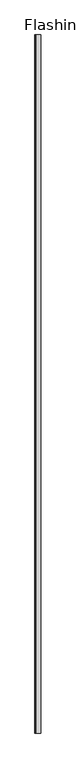
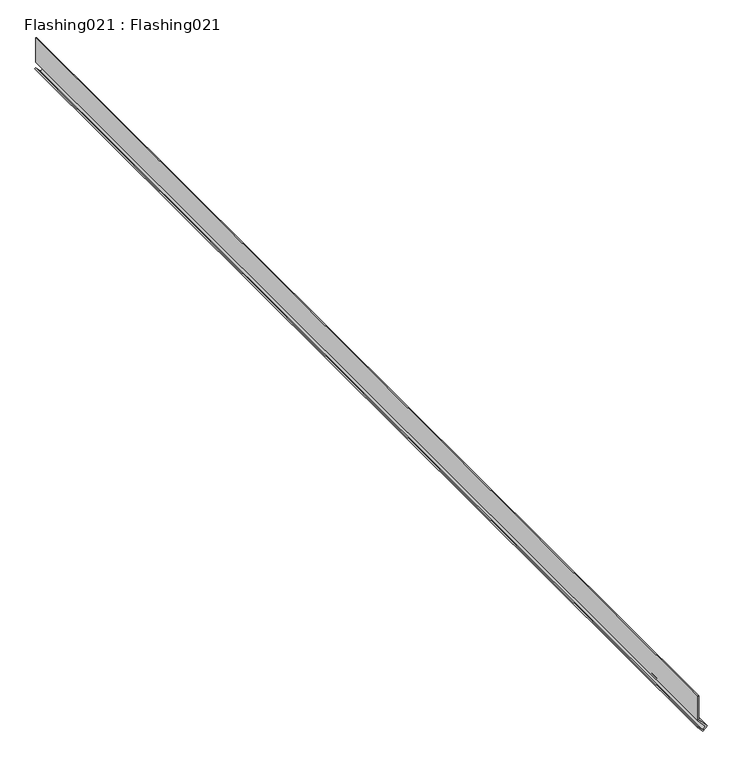
"""IFC4 building model written with IfcOpenShell, lengths in millimetres: proxy geometry, Flashing021 : Flashing021."""

import ifcopenshell
import ifcopenshell.guid

model = None  # the IFC model being written
_history = None  # IfcOwnerHistory: only IFC2X3 demands one
_inside = {}  # id of a spatial element -> (the spatial element, [elements in it])
_under = {}  # id of a project, library or spatial element -> (it, [spatial elements below it])
_declared = {}  # id of a project -> (the project, [libraries it declares])
_typed = {}  # id of a type object -> (the type object, [elements of that type])
_made_of = {}  # id of a material, layer set ... -> (it, [elements and type objects made of it])


def new_model(schema):
    """Start an empty IFC model of exactly this schema.

    Asked for "IFC4X3", IfcOpenShell would pick the latest addendum, in which some entities
    have other attributes; the version numbers below select the first issue.
    IFC2X3 requires an IfcOwnerHistory on every rooted entity: one is made here for all.
    """
    global model, _history
    if schema == "IFC4X3":
        model = ifcopenshell.file(schema_version=(4, 3, 0, 0))
    else:
        model = ifcopenshell.file(schema=schema)
    _inside.clear()
    _under.clear()
    _declared.clear()
    _typed.clear()
    _made_of.clear()
    _history = None
    if model.schema == "IFC2X3":
        org = make("IfcOrganization", Name="unknown")
        user = make(
            "IfcPersonAndOrganization",
            ThePerson=make("IfcPerson", FamilyName="unknown"),
            TheOrganization=org,
        )
        app = make(
            "IfcApplication",
            ApplicationDeveloper=org,
            Version="unknown",
            ApplicationFullName="unknown",
            ApplicationIdentifier="unknown",
        )
        _history = make(
            "IfcOwnerHistory",
            OwningUser=user,
            OwningApplication=app,
            ChangeAction="ADDED",
            CreationDate=0,
        )
    return model


def make(cls, **values):
    """One entity of the class cls with the attributes given. An attribute that is None is left unset."""
    return model.create_entity(
        cls, **{name: value for name, value in values.items() if value is not None}
    )


def rooted(cls, **values):
    """An entity with a GlobalId (a new one), such as an element, a storey or a relation."""
    return make(cls, GlobalId=ifcopenshell.guid.new(), OwnerHistory=_history, **values)


def si_unit(unit_type, name, prefix=None):
    """IfcSIUnit, for example si_unit("LENGTHUNIT", "METRE", prefix="MILLI")."""
    return make("IfcSIUnit", UnitType=unit_type, Prefix=prefix, Name=name)


def assignment(units):
    """IfcUnitAssignment: the units of a project."""
    return None if units is None else make("IfcUnitAssignment", Units=units)


def point(xyz):
    """IfcCartesianPoint."""
    return None if xyz is None else make("IfcCartesianPoint", Coordinates=xyz)


def direction(xyz):
    """IfcDirection."""
    return None if xyz is None else make("IfcDirection", DirectionRatios=xyz)


def frame(location, z_axis=None, x_axis=None):
    """IfcAxis2Placement3D, a coordinate frame: its origin and axes. An axis left out is left unset."""
    return make(
        "IfcAxis2Placement3D",
        Location=point(location),
        Axis=direction(z_axis),
        RefDirection=direction(x_axis),
    )


def origin():
    """The frame at (0, 0, 0) with its axes left unset."""
    return frame((0.0, 0.0, 0.0))


def place(relative_to, where):
    """IfcLocalPlacement: puts the frame where relative to a parent placement (None: the world)."""
    return make(
        "IfcLocalPlacement", PlacementRelTo=relative_to, RelativePlacement=where
    )


def context(
    kind, dimensions, precision=None, world=None, true_north=None, identifier=None
):
    """IfcGeometricRepresentationContext, for example the 3D "Model" context."""
    return make(
        "IfcGeometricRepresentationContext",
        ContextIdentifier=identifier,
        ContextType=kind,
        CoordinateSpaceDimension=dimensions,
        Precision=precision,
        WorldCoordinateSystem=world,
        TrueNorth=true_north,
    )


def project(units=None, contexts=None):
    """IfcProject with its units and contexts."""
    return rooted(
        "IfcProject",
        Name="project",
        RepresentationContexts=contexts,
        UnitsInContext=assignment(units),
    )


def spatial(cls, under=None, at=None, **own):
    """A site, building, storey or space (cls), placed at a placement, below another one or the project."""
    s = rooted(cls, ObjectPlacement=at, **own)
    if under is not None:
        _under.setdefault(under.id(), (under, []))[1].append(s)
    return s


def polyline(points):
    """IfcPolyline through the points."""
    return make("IfcPolyline", Points=[point(p) for p in points])


def outline(outer, holes=None, kind="AREA"):
    """IfcArbitraryClosedProfileDef: a profile drawn as a closed curve; with holes, ...WithVoids."""
    if holes is None:
        return make("IfcArbitraryClosedProfileDef", ProfileType=kind, OuterCurve=outer)
    return make(
        "IfcArbitraryProfileDefWithVoids",
        ProfileType=kind,
        OuterCurve=outer,
        InnerCurves=holes,
    )


def extrude(swept, where, along, depth):
    """IfcExtrudedAreaSolid: the profile swept, set in the frame where, extruded along a direction by depth."""
    return make(
        "IfcExtrudedAreaSolid",
        SweptArea=swept,
        Position=where,
        ExtrudedDirection=direction(along),
        Depth=depth,
    )


def shape(context_of_items, identifier, shape_type, items):
    """IfcShapeRepresentation: the items that make up one representation, for example the "Body"."""
    return make(
        "IfcShapeRepresentation",
        ContextOfItems=context_of_items,
        RepresentationIdentifier=identifier,
        RepresentationType=shape_type,
        Items=items,
    )


def source(mapping_origin, context_of_items, identifier, shape_type, items):
    """IfcRepresentationMap: a shape defined once, which mapped items show again and again."""
    return make(
        "IfcRepresentationMap",
        MappingOrigin=mapping_origin,
        MappedRepresentation=shape(context_of_items, identifier, shape_type, items),
    )


def transform(
    local_origin,
    x_axis=None,
    y_axis=None,
    z_axis=None,
    scale=None,
    scale2=None,
    scale3=None,
    uniform=True,
):
    """IfcCartesianTransformationOperator3D, or its non-uniform kind. x_axis, y_axis, z_axis: its Axis1, 2, 3."""
    if uniform:
        return make(
            "IfcCartesianTransformationOperator3D",
            Axis1=direction(x_axis),
            Axis2=direction(y_axis),
            LocalOrigin=point(local_origin),
            Scale=scale,
            Axis3=direction(z_axis),
        )
    return make(
        "IfcCartesianTransformationOperator3DnonUniform",
        Axis1=direction(x_axis),
        Axis2=direction(y_axis),
        LocalOrigin=point(local_origin),
        Scale=scale,
        Axis3=direction(z_axis),
        Scale2=scale2,
        Scale3=scale3,
    )


def mapped(mapping_source, mapping_target):
    """IfcMappedItem: shows the shape of a source again, moved by a transform."""
    return make(
        "IfcMappedItem", MappingSource=mapping_source, MappingTarget=mapping_target
    )


def made_of(thing, what):
    """Note that an element or type object is made of a material, layer set ...; save() writes the relation."""
    if what is not None:
        _made_of.setdefault(what.id(), (what, []))[1].append(thing)
    return thing


def element(
    cls,
    number,
    at=None,
    inside=None,
    cuts=None,
    type_object=None,
    material=None,
    context=None,
    identifier="Body",
    shape_type=None,
    held_by="IfcProductDefinitionShape",
    body=None,
    shapes=None,
    **own,
):
    """One element of the class cls, such as IfcWall. Its Tag is "e" and its number.

    at: its placement. inside: the storey or other place that contains it. cuts: it is an
    opening in that element (IfcRelVoidsElement). A single representation is given by context,
    identifier, shape_type and body (its items); several are given by shapes. held_by: the class
    of the entity that holds the representations. save() writes the other relations.
    """
    e = rooted(cls, Tag="e%d" % number, ObjectPlacement=at, **own)
    if body is not None:
        shapes = [shape(context, identifier, shape_type, body)]
    if shapes is not None:
        e.Representation = make(held_by, Representations=shapes)
    if inside is not None:
        _inside.setdefault(inside.id(), (inside, []))[1].append(e)
    if cuts is not None:
        rooted(
            "IfcRelVoidsElement", RelatingBuildingElement=cuts, RelatedOpeningElement=e
        )
    if type_object is not None:
        _typed.setdefault(type_object.id(), (type_object, []))[1].append(e)
    return made_of(e, material)


def aggregate(whole, parts):
    """IfcRelAggregates: a whole, such as a stair, and the parts it consists of."""
    return rooted("IfcRelAggregates", RelatingObject=whole, RelatedObjects=parts)


def save(model, path):
    """Write the relations noted so far, then the file.

    IfcRelAggregates (storeys below a building ...), IfcRelContainedInSpatialStructure (elements
    in a storey), IfcRelDefinesByType, IfcRelAssociatesMaterial and IfcRelDeclares: one each for
    every whole, place, type object, material and project.
    """
    for whole, parts in _under.values():
        aggregate(whole, parts)
    for where, things in _inside.values():
        rooted(
            "IfcRelContainedInSpatialStructure",
            RelatedElements=things,
            RelatingStructure=where,
        )
    for kind, things in _typed.values():
        rooted("IfcRelDefinesByType", RelatedObjects=things, RelatingType=kind)
    for what, things in _made_of.values():
        rooted("IfcRelAssociatesMaterial", RelatedObjects=things, RelatingMaterial=what)
    for by, libraries in _declared.values():
        rooted("IfcRelDeclares", RelatingContext=by, RelatedDefinitions=libraries)
    model.write(path)


def flashing021_flashing021_f64f48d8(model_context):
    return source(origin(), model_context, "Body", "SweptSolid", [
        extrude(outline(polyline([(43008.8710938, 16651.7480469), (42993.6445313, 16665.2148438), (42989.0546875, 16660.4316406), (42998.2304688, 16652.1347656), (42996.8890886, 16650.6512902), (42986.1852076, 16660.3298953), (42993.5310498, 16667.9852007), (43009.6286352, 16653.7480469), (43053.53125, 16653.7480469), (43053.53125, 16651.7480469), (43008.8710938, 16651.7480469)])), frame((0.0, 7982.1435673, 0.0), z_axis=(0.0, 1.0, 0.0), x_axis=(0.0, 0.0, 1.0)), (0.0, 0.0, 1.0), 2000.0),
    ])


if __name__ == "__main__":
    model = new_model("IFC4")
    model_context = context("Model", 3, world=origin())
    ifc_project = project(units=[si_unit("LENGTHUNIT", "METRE", prefix="MILLI")], contexts=[model_context])
    site = spatial("IfcSite", under=ifc_project)
    building = spatial("IfcBuilding", under=site)
    placement = place(None, origin())
    flashing021_flashing021_shape = flashing021_flashing021_f64f48d8(model_context)
    element("IfcBuildingElementProxy", 1, Name="Flashing021 : Flashing021", ObjectType="Flashing021 : Flashing021", at=placement, inside=building, context=model_context, shape_type="MappedRepresentation", body=[
        mapped(flashing021_flashing021_shape, transform((0.0, 0.0, 0.0), x_axis=(1.0, 0.0, 0.0), y_axis=(0.0, 1.0, 0.0), z_axis=(0.0, 0.0, 1.0))),
    ])
    save(model, "model.ifc")

# Revit data of these elements
# Type "Flashing021 : Flashing021"
#   NameOverride = "Flashing021"
# Element 1 (IfcBuildingElementProxy, "Flashing021 : Flashing021")
#   Materials on its faces: "16GA. COPPER BRAKE METAL FLASHING"
# Materials
#   "16GA. COPPER BRAKE METAL FLASHING": class "Unassigned", colour RGB 128 128 128, transparency 0, Cost = 0
